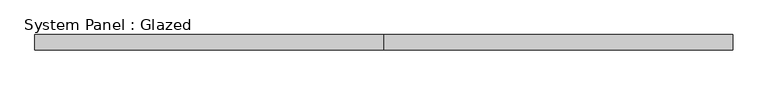
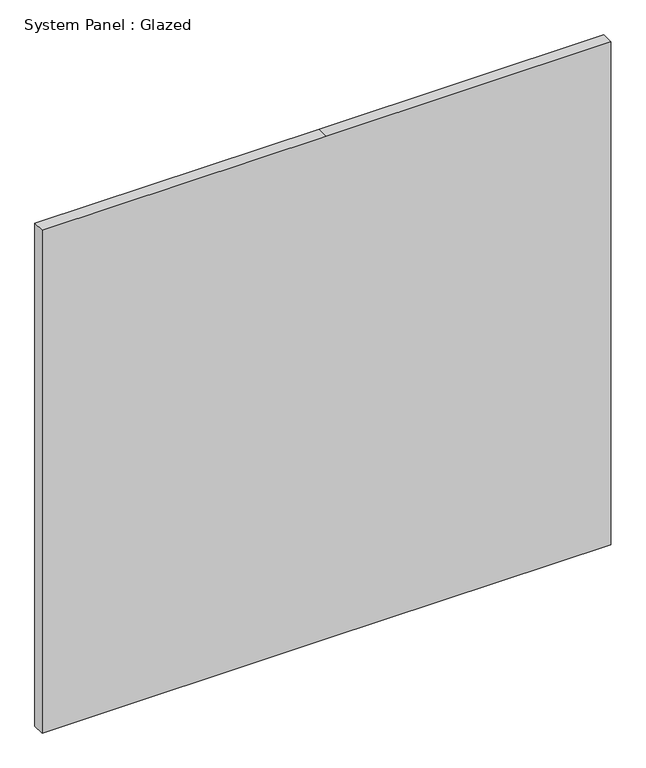
"""IFC4 building model written with IfcOpenShell, lengths in millimetres: plate geometry, System Panel : Glazed."""

from ifc_helpers import new_model, si_unit, frame, origin, place, context, project, spatial, polyline, outline, extrude, source, transform, mapped, element, save


def system_panel_glazed_aaf472d8(model_context):
    return source(origin(), model_context, "Body", "SweptSolid", [
        extrude(outline(polyline([(0.0, -1150.0), (0.0, 0.0), (0.0, 1150.0), (2150.0, 1150.0), (2150.0, 0.0), (2150.0, -1150.0), (0.0, -1150.0)])), frame((0.0, -25.0, 0.0), z_axis=(0.0, 1.0, 0.0), x_axis=(0.0, 0.0, 1.0)), (0.0, 0.0, 1.0), 50.0),
    ])


if __name__ == "__main__":
    model = new_model("IFC4")
    model_context = context("Model", 3, world=origin())
    ifc_project = project(units=[si_unit("LENGTHUNIT", "METRE", prefix="MILLI")], contexts=[model_context])
    site = spatial("IfcSite", under=ifc_project)
    building = spatial("IfcBuilding", under=site)
    placement = place(None, origin())
    system_panel_glazed_shape = system_panel_glazed_aaf472d8(model_context)
    element("IfcPlate", 1, ObjectType="System Panel : Glazed", at=placement, inside=building, context=model_context, shape_type="MappedRepresentation", body=[
        mapped(system_panel_glazed_shape, transform((0.0, 0.0, 0.0), x_axis=(1.0, 0.0, 0.0), y_axis=(0.0, 1.0, 0.0), z_axis=(0.0, 0.0, 1.0))),
    ])
    save(model, "model.ifc")

# Revit data of these elements
# Type "System Panel : Glazed"
#   Type Mark = "CW-GLASS"
# Element 1 (IfcPlate, "System Panel : Glazed")
#   Materials on its faces: "Glass_Clear"
# Materials
#   "Glass_Clear": class "Glass", colour RGB 128 128 255, transparency 0.8, Comments = "Rendering appearance not upgraded ", Cost = 0
